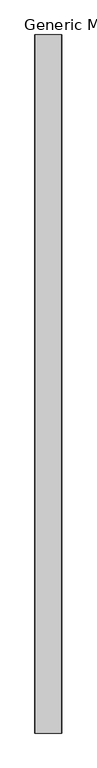
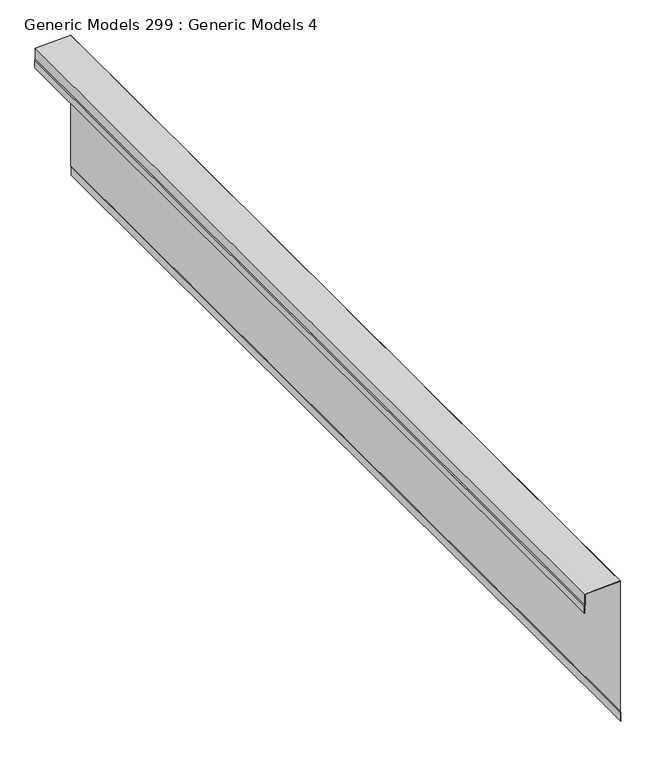
"""IFC4 building model written with IfcOpenShell, lengths in millimetres: proxy geometry, Generic Models 299 : Generic Models 4."""

from ifc_helpers import new_model, si_unit, frame, origin, place, context, project, spatial, polyline, outline, extrude, source, transform, mapped, element, save


def generic_models_299_generic_models_4_91095fc9(model_context):
    return source(origin(), model_context, "Body", "SweptSolid", [
        extrude(outline(polyline([(127013.3250789, 8389.1524314), (127020.4570194, 8391.7482454), (127078.1640881, 8391.7482454), (127085.7438493, 8573.6625161), (126373.0569671, 8573.6625161), (126363.2827828, 8577.2200282), (126319.1058133, 8577.2200282), (126319.1058133, 8578.1054172), (126363.1709664, 8578.1054172), (126373.1969267, 8574.4562661), (127086.571361, 8574.4562661), (127078.9254539, 8390.9544954), (127020.596979, 8390.9544954), (127013.4650384, 8388.3586814), (126974.0744351, 8388.3586814), (126974.0744351, 8389.1524314), (127013.3250789, 8389.1524314)])), frame((0.0, 6851.0769662, 0.0), z_axis=(0.0, 1.0, 0.0), x_axis=(0.0, 0.0, 1.0)), (0.0, 0.0, 1.0), 4927.6),
    ])


if __name__ == "__main__":
    model = new_model("IFC4")
    model_context = context("Model", 3, world=origin())
    ifc_project = project(units=[si_unit("LENGTHUNIT", "METRE", prefix="MILLI")], contexts=[model_context])
    site = spatial("IfcSite", under=ifc_project)
    building = spatial("IfcBuilding", under=site)
    placement = place(None, origin())
    generic_models_299_generic_models_4_shape = generic_models_299_generic_models_4_91095fc9(model_context)
    element("IfcBuildingElementProxy", 1, Name="Generic Models 299 : Generic Models 4", ObjectType="Generic Models 299 : Generic Models 4", at=placement, inside=building, context=model_context, shape_type="MappedRepresentation", body=[
        mapped(generic_models_299_generic_models_4_shape, transform((0.0, 0.0, 0.0), x_axis=(1.0, 0.0, 0.0), y_axis=(0.0, 1.0, 0.0), z_axis=(0.0, 0.0, 1.0))),
    ])
    save(model, "model.ifc")

# Revit data of these elements
# Element 1 (IfcBuildingElementProxy, "Generic Models 299 : Generic Models 4")
#   Materials on its faces: "_(2) LAYERS NO. 30 ASTM D226 ASPHALT SATURATED ORGANIC FELT"
# Materials
#   "_(2) LAYERS NO. 30 ASTM D226 ASPHALT SATURATED ORGANIC FELT": class "Generic", colour RGB 67 154 161, transparency 0, Cost = 0
